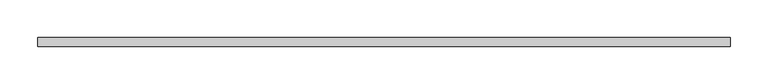
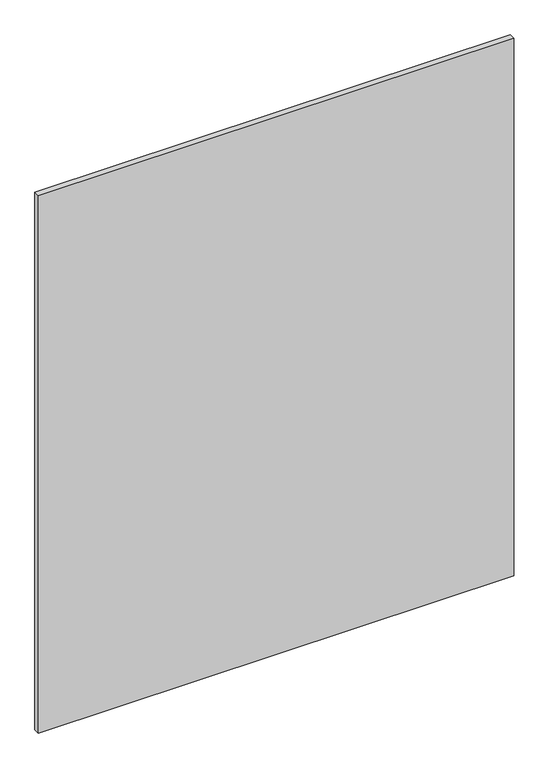
"""IFC4 building model written with IfcOpenShell, lengths in millimetres: railing geometry, ML_Painéis4 : ML_Painéis."""

import ifcopenshell
import ifcopenshell.guid

model = None  # the IFC model being written
_history = None  # IfcOwnerHistory: only IFC2X3 demands one
_inside = {}  # id of a spatial element -> (the spatial element, [elements in it])
_under = {}  # id of a project, library or spatial element -> (it, [spatial elements below it])
_declared = {}  # id of a project -> (the project, [libraries it declares])
_typed = {}  # id of a type object -> (the type object, [elements of that type])
_made_of = {}  # id of a material, layer set ... -> (it, [elements and type objects made of it])


def new_model(schema):
    """Start an empty IFC model of exactly this schema.

    Asked for "IFC4X3", IfcOpenShell would pick the latest addendum, in which some entities
    have other attributes; the version numbers below select the first issue.
    IFC2X3 requires an IfcOwnerHistory on every rooted entity: one is made here for all.
    """
    global model, _history
    if schema == "IFC4X3":
        model = ifcopenshell.file(schema_version=(4, 3, 0, 0))
    else:
        model = ifcopenshell.file(schema=schema)
    _inside.clear()
    _under.clear()
    _declared.clear()
    _typed.clear()
    _made_of.clear()
    _history = None
    if model.schema == "IFC2X3":
        org = make("IfcOrganization", Name="unknown")
        user = make(
            "IfcPersonAndOrganization",
            ThePerson=make("IfcPerson", FamilyName="unknown"),
            TheOrganization=org,
        )
        app = make(
            "IfcApplication",
            ApplicationDeveloper=org,
            Version="unknown",
            ApplicationFullName="unknown",
            ApplicationIdentifier="unknown",
        )
        _history = make(
            "IfcOwnerHistory",
            OwningUser=user,
            OwningApplication=app,
            ChangeAction="ADDED",
            CreationDate=0,
        )
    return model


def make(cls, **values):
    """One entity of the class cls with the attributes given. An attribute that is None is left unset."""
    return model.create_entity(
        cls, **{name: value for name, value in values.items() if value is not None}
    )


def rooted(cls, **values):
    """An entity with a GlobalId (a new one), such as an element, a storey or a relation."""
    return make(cls, GlobalId=ifcopenshell.guid.new(), OwnerHistory=_history, **values)


def si_unit(unit_type, name, prefix=None):
    """IfcSIUnit, for example si_unit("LENGTHUNIT", "METRE", prefix="MILLI")."""
    return make("IfcSIUnit", UnitType=unit_type, Prefix=prefix, Name=name)


def assignment(units):
    """IfcUnitAssignment: the units of a project."""
    return None if units is None else make("IfcUnitAssignment", Units=units)


def point(xyz):
    """IfcCartesianPoint."""
    return None if xyz is None else make("IfcCartesianPoint", Coordinates=xyz)


def direction(xyz):
    """IfcDirection."""
    return None if xyz is None else make("IfcDirection", DirectionRatios=xyz)


def frame(location, z_axis=None, x_axis=None):
    """IfcAxis2Placement3D, a coordinate frame: its origin and axes. An axis left out is left unset."""
    return make(
        "IfcAxis2Placement3D",
        Location=point(location),
        Axis=direction(z_axis),
        RefDirection=direction(x_axis),
    )


def origin():
    """The frame at (0, 0, 0) with its axes left unset."""
    return frame((0.0, 0.0, 0.0))


def place(relative_to, where):
    """IfcLocalPlacement: puts the frame where relative to a parent placement (None: the world)."""
    return make(
        "IfcLocalPlacement", PlacementRelTo=relative_to, RelativePlacement=where
    )


def context(
    kind, dimensions, precision=None, world=None, true_north=None, identifier=None
):
    """IfcGeometricRepresentationContext, for example the 3D "Model" context."""
    return make(
        "IfcGeometricRepresentationContext",
        ContextIdentifier=identifier,
        ContextType=kind,
        CoordinateSpaceDimension=dimensions,
        Precision=precision,
        WorldCoordinateSystem=world,
        TrueNorth=true_north,
    )


def project(units=None, contexts=None):
    """IfcProject with its units and contexts."""
    return rooted(
        "IfcProject",
        Name="project",
        RepresentationContexts=contexts,
        UnitsInContext=assignment(units),
    )


def spatial(cls, under=None, at=None, **own):
    """A site, building, storey or space (cls), placed at a placement, below another one or the project."""
    s = rooted(cls, ObjectPlacement=at, **own)
    if under is not None:
        _under.setdefault(under.id(), (under, []))[1].append(s)
    return s


def polyline(points):
    """IfcPolyline through the points."""
    return make("IfcPolyline", Points=[point(p) for p in points])


def outline(outer, holes=None, kind="AREA"):
    """IfcArbitraryClosedProfileDef: a profile drawn as a closed curve; with holes, ...WithVoids."""
    if holes is None:
        return make("IfcArbitraryClosedProfileDef", ProfileType=kind, OuterCurve=outer)
    return make(
        "IfcArbitraryProfileDefWithVoids",
        ProfileType=kind,
        OuterCurve=outer,
        InnerCurves=holes,
    )


def extrude(swept, where, along, depth):
    """IfcExtrudedAreaSolid: the profile swept, set in the frame where, extruded along a direction by depth."""
    return make(
        "IfcExtrudedAreaSolid",
        SweptArea=swept,
        Position=where,
        ExtrudedDirection=direction(along),
        Depth=depth,
    )


def shape(context_of_items, identifier, shape_type, items):
    """IfcShapeRepresentation: the items that make up one representation, for example the "Body"."""
    return make(
        "IfcShapeRepresentation",
        ContextOfItems=context_of_items,
        RepresentationIdentifier=identifier,
        RepresentationType=shape_type,
        Items=items,
    )


def source(mapping_origin, context_of_items, identifier, shape_type, items):
    """IfcRepresentationMap: a shape defined once, which mapped items show again and again."""
    return make(
        "IfcRepresentationMap",
        MappingOrigin=mapping_origin,
        MappedRepresentation=shape(context_of_items, identifier, shape_type, items),
    )


def transform(
    local_origin,
    x_axis=None,
    y_axis=None,
    z_axis=None,
    scale=None,
    scale2=None,
    scale3=None,
    uniform=True,
):
    """IfcCartesianTransformationOperator3D, or its non-uniform kind. x_axis, y_axis, z_axis: its Axis1, 2, 3."""
    if uniform:
        return make(
            "IfcCartesianTransformationOperator3D",
            Axis1=direction(x_axis),
            Axis2=direction(y_axis),
            LocalOrigin=point(local_origin),
            Scale=scale,
            Axis3=direction(z_axis),
        )
    return make(
        "IfcCartesianTransformationOperator3DnonUniform",
        Axis1=direction(x_axis),
        Axis2=direction(y_axis),
        LocalOrigin=point(local_origin),
        Scale=scale,
        Axis3=direction(z_axis),
        Scale2=scale2,
        Scale3=scale3,
    )


def mapped(mapping_source, mapping_target):
    """IfcMappedItem: shows the shape of a source again, moved by a transform."""
    return make(
        "IfcMappedItem", MappingSource=mapping_source, MappingTarget=mapping_target
    )


def made_of(thing, what):
    """Note that an element or type object is made of a material, layer set ...; save() writes the relation."""
    if what is not None:
        _made_of.setdefault(what.id(), (what, []))[1].append(thing)
    return thing


def element(
    cls,
    number,
    at=None,
    inside=None,
    cuts=None,
    type_object=None,
    material=None,
    context=None,
    identifier="Body",
    shape_type=None,
    held_by="IfcProductDefinitionShape",
    body=None,
    shapes=None,
    **own,
):
    """One element of the class cls, such as IfcWall. Its Tag is "e" and its number.

    at: its placement. inside: the storey or other place that contains it. cuts: it is an
    opening in that element (IfcRelVoidsElement). A single representation is given by context,
    identifier, shape_type and body (its items); several are given by shapes. held_by: the class
    of the entity that holds the representations. save() writes the other relations.
    """
    e = rooted(cls, Tag="e%d" % number, ObjectPlacement=at, **own)
    if body is not None:
        shapes = [shape(context, identifier, shape_type, body)]
    if shapes is not None:
        e.Representation = make(held_by, Representations=shapes)
    if inside is not None:
        _inside.setdefault(inside.id(), (inside, []))[1].append(e)
    if cuts is not None:
        rooted(
            "IfcRelVoidsElement", RelatingBuildingElement=cuts, RelatedOpeningElement=e
        )
    if type_object is not None:
        _typed.setdefault(type_object.id(), (type_object, []))[1].append(e)
    return made_of(e, material)


def aggregate(whole, parts):
    """IfcRelAggregates: a whole, such as a stair, and the parts it consists of."""
    return rooted("IfcRelAggregates", RelatingObject=whole, RelatedObjects=parts)


def save(model, path):
    """Write the relations noted so far, then the file.

    IfcRelAggregates (storeys below a building ...), IfcRelContainedInSpatialStructure (elements
    in a storey), IfcRelDefinesByType, IfcRelAssociatesMaterial and IfcRelDeclares: one each for
    every whole, place, type object, material and project.
    """
    for whole, parts in _under.values():
        aggregate(whole, parts)
    for where, things in _inside.values():
        rooted(
            "IfcRelContainedInSpatialStructure",
            RelatedElements=things,
            RelatingStructure=where,
        )
    for kind, things in _typed.values():
        rooted("IfcRelDefinesByType", RelatedObjects=things, RelatingType=kind)
    for what, things in _made_of.values():
        rooted("IfcRelAssociatesMaterial", RelatedObjects=things, RelatingMaterial=what)
    for by, libraries in _declared.values():
        rooted("IfcRelDeclares", RelatingContext=by, RelatedDefinitions=libraries)
    model.write(path)


def railing_29f9e2f6(model_context):
    return source(origin(), model_context, "Body", "SweptSolid", [
        extrude(outline(polyline([(-4674.5702584, 2133.3602771), (-4674.5702584, 2121.3602771), (-5595.5702584, 2121.3602771), (-5595.5702584, 2133.3602771), (-4674.5702584, 2133.3602771)])), frame((0.0, 0.0, 4122.0679199), z_axis=(0.0, 0.0, 1.0), x_axis=(1.0, 0.0, 0.0)), (0.0, 0.0, 1.0), 1100.0),
    ])


if __name__ == "__main__":
    model = new_model("IFC4")
    model_context = context("Model", 3, world=origin())
    ifc_project = project(units=[si_unit("LENGTHUNIT", "METRE", prefix="MILLI")], contexts=[model_context])
    site = spatial("IfcSite", under=ifc_project)
    building = spatial("IfcBuilding", under=site)
    placement = place(None, origin())
    railing_shape = railing_29f9e2f6(model_context)
    element("IfcRailing", 1, ObjectType="ML_Painéis4 : ML_Painéis", at=placement, inside=building, context=model_context, shape_type="MappedRepresentation", body=[
        mapped(railing_shape, transform((0.0, 0.0, 0.0), x_axis=(1.0, 0.0, 0.0), y_axis=(0.0, 1.0, 0.0), z_axis=(0.0, 0.0, 1.0))),
    ])
    save(model, "model.ifc")

# Revit data of these elements
# Type "ML_Painéis4 : ML_Painéis"
#   ME_Área [instance default] = 1.0131 m²
#   ME_Espessura [instance default] = 0.012 m
#   ME_Dist Painéis [instance default] = 0.002 m
#   ME_Compr Painéis [instance default] = 0.921 m
#   ME_Compr [instance default] = 0.925 m
#   ME_Altura [instance default] = 1.10 m
#   ME_Quant Painéis [instance default] = 3
#   ME_Painel Único [instance default] = yes
#   ME_Paineis Vários [instance default] = no
#   ME_Material Tipo Vidro [instance default] = .VIDRO GENÉRICO
# Element 1 (IfcRailing, "ML_Painéis4 : ML_Painéis")
#   Materials on its faces: ".VIDRO GENÉRICO"
# Materials
#   ".VIDRO GENÉRICO": class ".CC_VIDRO", colour RGB 0 128 192, transparency 0.9, Description = "Vidro comum", Cost = 0
